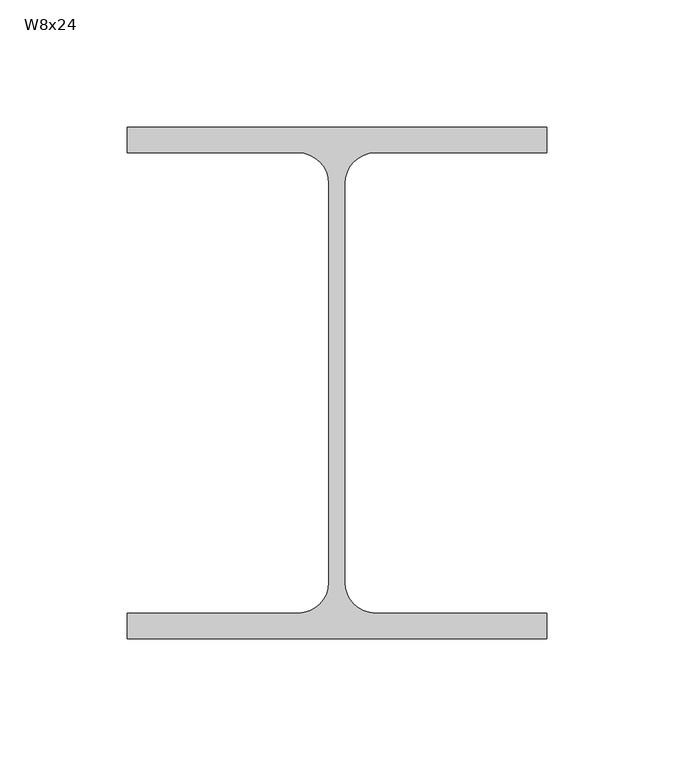
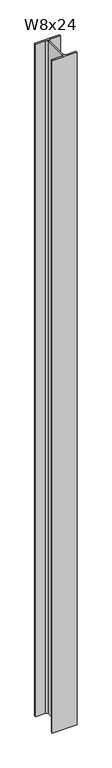
"""IFC4 building model written with IfcOpenShell, lengths in millimetres: column geometry, RME WF - Column : W8x24."""

from ifc_helpers import new_model, si_unit, point, frame, frame_2d, origin, place, context, project, spatial, polyline, circle_curve, trimmed, segment, composite_curve, outline, extrude, source, transform, mapped, element, save


def w8x24_0742124d(model_context):
    return source(origin(), model_context, "Body", "SweptSolid", [
        extrude(outline(composite_curve([segment(polyline([(82.55, 100.711), (82.55, 90.551), (15.1765, 90.551)]), True, "CONTINUOUS"), segment(trimmed(circle_curve(frame_2d((15.1765, 78.486)), 12.065), [point((15.1765, 90.551))], [point((3.1115, 78.486))], True, "CARTESIAN"), True, "CONTINUOUS"), segment(polyline([(3.1115, 78.486), (3.1115, -78.486)]), True, "CONTINUOUS"), segment(trimmed(circle_curve(frame_2d((15.1765, -78.486)), 12.065), [point((3.1115, -78.486))], [point((15.1765, -90.551))], True, "CARTESIAN"), True, "CONTINUOUS"), segment(polyline([(15.1765, -90.551), (82.55, -90.551), (82.55, -100.711), (-82.55, -100.711), (-82.55, -90.551), (-15.1765, -90.551)]), True, "CONTINUOUS"), segment(trimmed(circle_curve(frame_2d((-15.1765, -78.486)), 12.065), [point((-15.1765, -90.551))], [point((-3.1115, -78.486))], True, "CARTESIAN"), True, "CONTINUOUS"), segment(polyline([(-3.1115, -78.486), (-3.1115, 78.486)]), True, "CONTINUOUS"), segment(trimmed(circle_curve(frame_2d((-15.1765, 78.486)), 12.065), [point((-3.1115, 78.486))], [point((-15.1765, 90.551))], True, "CARTESIAN"), True, "CONTINUOUS"), segment(polyline([(-15.1765, 90.551), (-82.55, 90.551), (-82.55, 100.711), (82.55, 100.711)]), True, "CONTINUOUS")], self_intersect=False)), frame((0.0, 0.0, -304.8), z_axis=(0.0, 0.0, 1.0), x_axis=(1.0, 0.0, 0.0)), (0.0, 0.0, 1.0), 4727.575),
    ])


if __name__ == "__main__":
    model = new_model("IFC4")
    model_context = context("Model", 3, world=origin())
    ifc_project = project(units=[si_unit("LENGTHUNIT", "METRE", prefix="MILLI")], contexts=[model_context])
    site = spatial("IfcSite", under=ifc_project)
    building = spatial("IfcBuilding", under=site)
    placement = place(None, origin())
    w8x24_shape = w8x24_0742124d(model_context)
    element("IfcColumn", 1, ObjectType="RME WF - Column : W8x24", at=placement, inside=building, context=model_context, shape_type="MappedRepresentation", body=[
        mapped(w8x24_shape, transform((0.0, 0.0, 0.0), x_axis=(1.0, 0.0, 0.0), y_axis=(0.0, 1.0, 0.0), z_axis=(0.0, 0.0, 1.0))),
    ])
    save(model, "model.ifc")

# Revit data of these elements
# Type "RME WF - Column : W8x24"
#   Type Mark = "C1"
#   REINF TYPE [instance default] = ""
#   Nominal Size = "W16"
#   COL REMARKS [instance default] = ""
#   BP [instance default] = ""
#   Assembly Code = "B10"
#   W = 24
#   bf = 0' - 6 1/2"
#   d = 0' - 7.93"
#   k = 0' - 0 7/8"
#   kr = 0' - 0.475"
#   tf = 0' - 0.4"
#   tw = 0' - 0.245"
#   A = 0.0491667 SF
#   Structural Material [instance default] = Metal - Steel - ASTM A992
# Element 1 (IfcColumn, "RME WF - Column : W8x24")
#   Materials on its faces: "Metal - Steel - ASTM A992"
# Materials
#   "Metal - Steel - ASTM A992": class "Metal", colour RGB 255 128 0, transparency 0
